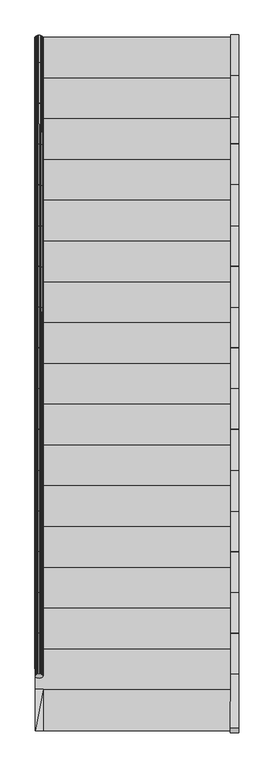
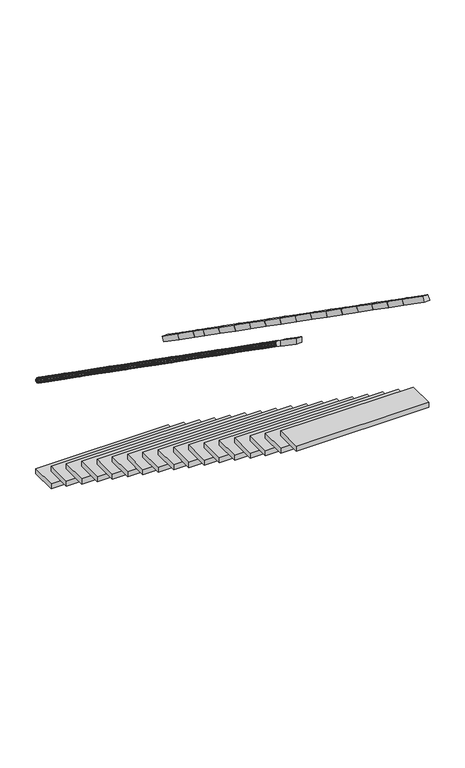
"""IFC4 building model written with IfcOpenShell, lengths in millimetres: stair geometry, 0_3d."""

from ifc_helpers import new_model, si_unit, frame, origin, origin_with_axes, place, context, project, spatial, polyline, outline, extrude, faceted_brep, source, transform, mapped, element, save


def stair_8f8480cc(model_context):
    return source(origin(), model_context, "Body", "SolidModel", [
        extrude(outline(polyline([(8.0820225, -49.3424859), (0.0, 0.0), (301.246492, 49.3424859), (309.3285145, 0.0), (8.0820225, -49.3424859)])), frame((1249.6426286, 1832.7635324, 2592.2240094), z_axis=(8.41828831730923e-05, 0.5732803643846047, 0.8193592720683017), x_axis=(-0.16175918326000965, -0.8085607216158117, 0.5657415718251334)), (0.0, 0.0, 1.0), 50.0),
        extrude(outline(polyline([(1249.9265282, 3766.1029394), (1249.8897991, 3515.9797843), (0.1101896, 3516.5348933), (0.0734597, 3766.4117944), (1249.9265282, 3766.1029394)])), frame((0.0, 0.0, 350.0), z_axis=(0.0, 0.0, 1.0), x_axis=(1.0, 0.0, 0.0)), (0.0, 0.0, 1.0), 50.0),
        faceted_brep([(1.5427287, 2095.0138491, 2432.7450302), (0.3185352, 2099.1390121, 2438.6355957), (1.5415159, 2103.2645348, 2444.5261612), (5.0919569, 2106.9865824, 2449.8401171), (10.6223163, 2109.9408148, 2454.0572963), (17.5912439, 2111.8380512, 2456.7648921), (25.3165726, 2112.4925769, 2457.697866), (33.0420935, 2111.8403223, 2456.7648921), (40.0115786, 2109.9451348, 2454.0572963), (45.5428062, 2106.9925283, 2449.8401171), (49.0943412, 2103.2715247, 2444.5261612), (50.3185347, 2099.1463617, 2438.6355957), (49.095554, 2095.0208389, 2432.7450302), (45.545113, 2091.2987914, 2427.4310744), (40.0147537, 2088.344559, 2423.2138951), (33.045826, 2086.4473226, 2420.5062993), (25.3204973, 2085.7927969, 2419.5733254), (17.5949765, 2086.4450514, 2420.5062993), (10.6254914, 2088.340239, 2423.2138951), (5.0942637, 2091.2928454, 2427.4310744), (0.3552659, 1849.2569855, 2613.6356001), (1.5782465, 1853.3825079, 2619.5261658), (5.1286875, 1857.1045552, 2624.8401219), (10.6590469, 1860.0587874, 2629.0573013), (17.6279745, 1861.9560236, 2631.7648972), (25.3533033, 1862.6105493, 2632.6978712), (33.0788241, 1861.9582948, 2631.7648972), (40.0483092, 1860.0631074, 2629.0573013), (45.5795368, 1857.1105012, 2624.8401219), (49.1310718, 1853.3894978, 2619.5261658), (50.3552653, 1849.2643351, 2613.6356001), (49.1322846, 1845.1388127, 2607.7450345), (45.5818436, 1841.4167654, 2602.4310784), (40.0514843, 1838.4625333, 2598.213899), (33.0825566, 1836.565297, 2595.5063031), (25.3572279, 1835.9107713, 2594.5733291), (17.6317071, 1836.5630258, 2595.5063031), (10.662222, 1838.4582133, 2598.213899), (5.1309944, 1841.4108195, 2602.4310784), (1.5794593, 1845.1318228, 2607.7450345)], [[[0, 1, 2, 3, 4, 5, 6, 7, 8, 9, 10, 11, 12, 13, 14, 15, 16, 17, 18, 19]], [[2, 1, 20, 21]], [[3, 2, 21, 22]], [[4, 3, 22, 23]], [[5, 4, 23, 24]], [[6, 5, 24, 25]], [[7, 6, 25, 26]], [[8, 7, 26, 27]], [[9, 8, 27, 28]], [[10, 9, 28, 29]], [[11, 10, 29, 30]], [[12, 11, 30, 31]], [[13, 12, 31, 32]], [[14, 13, 32, 33]], [[15, 14, 33, 34]], [[16, 15, 34, 35]], [[17, 16, 35, 36]], [[18, 17, 36, 37]], [[19, 18, 37, 38]], [[0, 19, 38, 39]], [[1, 0, 39, 20]], [[21, 20, 39, 38, 37, 36, 35, 34, 33, 32, 31, 30, 29, 28, 27, 26, 25, 24, 23, 22]]]),
        extrude(outline(polyline([(1249.5959661, 1514.9945425), (1249.5592369, 1264.8713869), (0.4407586, 1267.6414831), (0.4040287, 1517.5186441), (1249.5959661, 1514.9945425)])), frame((0.0, 0.0, 1925.0), z_axis=(0.0, 0.0, 1.0), x_axis=(1.0, 0.0, 0.0)), (0.0, 0.0, 1.0), 50.0),
        extrude(outline(polyline([(1249.7061535, 2265.3640086), (1249.6694243, 2015.2408533), (0.3305689, 2017.2728797), (0.293839, 2267.1499541), (1249.7061535, 2265.3640086)])), frame((0.0, 0.0, 1400.0), z_axis=(0.0, 0.0, 1.0), x_axis=(1.0, 0.0, 0.0)), (0.0, 0.0, 1.0), 50.0),
        extrude(outline(polyline([(1249.6694243, 2015.2408533), (1249.6326952, 1765.1176979), (0.3672988, 1767.3957763), (0.3305689, 2017.2728797), (1249.6694243, 2015.2408533)])), frame((0.0, 0.0, 1575.0), z_axis=(0.0, 0.0, 1.0), x_axis=(1.0, 0.0, 0.0)), (0.0, 0.0, 1.0), 50.0),
        faceted_brep([(1.5794593, 1845.1318228, 2607.7450345), (0.3552659, 1849.2569855, 2613.6356001), (1.5782465, 1853.3825079, 2619.5261658), (5.1286875, 1857.1045552, 2624.8401219), (10.6590469, 1860.0587874, 2629.0573013), (17.6279745, 1861.9560236, 2631.7648972), (25.3533033, 1862.6105493, 2632.6978712), (33.0788241, 1861.9582948, 2631.7648972), (40.0483092, 1860.0631074, 2629.0573013), (45.5795368, 1857.1105012, 2624.8401219), (49.1310718, 1853.3894978, 2619.5261658), (50.3552653, 1849.2643351, 2613.6356001), (49.1322846, 1845.1388127, 2607.7450345), (45.5818436, 1841.4167654, 2602.4310784), (40.0514843, 1838.4625333, 2598.213899), (33.0825566, 1836.565297, 2595.5063031), (25.3572279, 1835.9107713, 2594.5733291), (17.6317071, 1836.5630258, 2595.5063031), (10.662222, 1838.4582133, 2598.213899), (5.1309944, 1841.4108195, 2602.4310784), (0.3919965, 1599.3749301, 2788.6356046), (1.6149772, 1603.5004522, 2794.5261705), (5.1654181, 1607.2224992, 2799.8401268), (10.6957775, 1610.1767311, 2804.0573064), (17.6647052, 1612.0739672, 2806.7649023), (25.3900339, 1612.7284928, 2807.6978763), (33.1155547, 1612.0762384, 2806.7649023), (40.0850398, 1610.1810511, 2804.0573064), (45.6162674, 1607.2284451, 2799.8401268), (49.1678025, 1603.5074421, 2794.5261705), (50.3919959, 1599.3822797, 2788.6356046), (49.1690153, 1595.2567576, 2782.7450387), (45.6185743, 1591.5347106, 2777.4310824), (40.0882149, 1588.5804787, 2773.2139028), (33.1192873, 1586.6832425, 2770.5063068), (25.3939585, 1586.0287169, 2769.5733329), (17.6684377, 1586.6809714, 2770.5063068), (10.6989526, 1588.5761587, 2773.2139028), (5.167725, 1591.5287647, 2777.4310824), (1.6161899, 1595.2497677, 2782.7450387)], [[[0, 1, 2, 3, 4, 5, 6, 7, 8, 9, 10, 11, 12, 13, 14, 15, 16, 17, 18, 19]], [[2, 1, 20, 21]], [[3, 2, 21, 22]], [[4, 3, 22, 23]], [[5, 4, 23, 24]], [[6, 5, 24, 25]], [[7, 6, 25, 26]], [[8, 7, 26, 27]], [[9, 8, 27, 28]], [[10, 9, 28, 29]], [[11, 10, 29, 30]], [[12, 11, 30, 31]], [[13, 12, 31, 32]], [[14, 13, 32, 33]], [[15, 14, 33, 34]], [[16, 15, 34, 35]], [[17, 16, 35, 36]], [[18, 17, 36, 37]], [[19, 18, 37, 38]], [[0, 19, 38, 39]], [[1, 0, 39, 20]], [[21, 20, 39, 38, 37, 36, 35, 34, 33, 32, 31, 30, 29, 28, 27, 26, 25, 24, 23, 22]]]),
        faceted_brep([(1.3223451, 3594.3053999, 1382.7450049), (0.0981516, 3598.4305649, 1388.635569), (1.3211323, 3602.5560896, 1394.5261331), (4.8715733, 3606.2781388, 1399.8400878), (10.4019326, 3609.2323726, 1404.0572661), (17.3708603, 3611.1296099, 1406.7648612), (25.096189, 3611.7841359, 1407.6978349), (32.8217098, 3611.1318811, 1406.7648612), (39.7911949, 3609.2366926, 1404.0572661), (45.3224225, 3606.2840848, 1399.8400878), (48.8739576, 3602.5630794, 1394.5261331), (50.0981511, 3598.4379145, 1388.635569), (48.8751704, 3594.3123898, 1382.7450049), (45.3247294, 3590.5903405, 1377.4310502), (39.79437, 3587.6361067, 1373.2138719), (32.8254424, 3585.7388695, 1370.5062768), (25.1001137, 3585.0843435, 1369.5733031), (17.3745928, 3585.7365983, 1370.5062768), (10.4051077, 3587.6317868, 1373.2138719), (4.8738801, 3590.5843946, 1377.4310502), (0.1348822, 3348.5487117, 1563.6355734), (1.3578629, 3352.674236, 1569.5261378), (4.9083039, 3356.396285, 1574.8400927), (10.4386632, 3359.3505186, 1579.0572711), (17.4075909, 3361.2477557, 1581.7648664), (25.1329196, 3361.9022817, 1582.6978401), (32.8584404, 3361.2500269, 1581.7648664), (39.8279255, 3359.3548385, 1579.0572711), (45.3591531, 3356.402231, 1574.8400927), (48.9106882, 3352.6812259, 1569.5261378), (50.1348816, 3348.5560613, 1563.6355734), (48.911901, 3344.4305369, 1557.7450091), (45.36146, 3340.7084879, 1552.4310542), (39.8311006, 3337.7542544, 1548.2138758), (32.862173, 3335.8570172, 1545.5062805), (25.1368442, 3335.2024913, 1544.5733068), (17.4113234, 3335.8547461, 1545.5062805), (10.4418383, 3337.7499344, 1548.2138758), (4.9106107, 3340.702542, 1552.4310542), (1.3590757, 3344.423547, 1557.7450091)], [[[0, 1, 2, 3, 4, 5, 6, 7, 8, 9, 10, 11, 12, 13, 14, 15, 16, 17, 18, 19]], [[2, 1, 20, 21]], [[3, 2, 21, 22]], [[4, 3, 22, 23]], [[5, 4, 23, 24]], [[6, 5, 24, 25]], [[7, 6, 25, 26]], [[8, 7, 26, 27]], [[9, 8, 27, 28]], [[10, 9, 28, 29]], [[11, 10, 29, 30]], [[12, 11, 30, 31]], [[13, 12, 31, 32]], [[14, 13, 32, 33]], [[15, 14, 33, 34]], [[16, 15, 34, 35]], [[17, 16, 35, 36]], [[18, 17, 36, 37]], [[19, 18, 37, 38]], [[0, 19, 38, 39]], [[1, 0, 39, 20]], [[21, 20, 39, 38, 37, 36, 35, 34, 33, 32, 31, 30, 29, 28, 27, 26, 25, 24, 23, 22]]]),
        faceted_brep([(1.4692675, 2594.7778149, 2082.7450218), (0.245074, 2598.9029786, 2088.6355868), (1.4680547, 2603.028502, 2094.5261518), (5.0184957, 2606.7505501, 2099.8401073), (10.548855, 2609.704783, 2104.0572862), (17.5177827, 2611.6020197, 2106.7648818), (25.2431114, 2612.2565455, 2107.6978556), (32.9686322, 2611.6042908, 2106.7648818), (39.9381173, 2609.709103, 2104.0572862), (45.4693449, 2606.7564961, 2099.8401073), (49.02088, 2603.0354919, 2094.5261518), (50.2450735, 2598.9103282, 2088.6355868), (49.0220928, 2594.7848048, 2082.7450218), (45.4716518, 2591.0627567, 2077.4310663), (39.9412924, 2588.1085238, 2073.2138874), (32.9723648, 2586.2112871, 2070.5062918), (25.2470361, 2585.5567613, 2069.573318), (17.5215152, 2586.209016, 2070.5062918), (10.5520301, 2588.1042038, 2073.2138874), (5.0208025, 2591.0568107, 2077.4310663), (0.2818046, 2349.0210098, 2263.6355913), (1.5047853, 2353.1465328, 2269.5261565), (5.0552263, 2356.8685807, 2274.8401122), (10.5855856, 2359.8228133, 2279.0572913), (17.5545133, 2361.7200499, 2281.7648869), (25.279842, 2362.3745756, 2282.6978608), (33.0053628, 2361.722321, 2281.7648869), (39.9748479, 2359.8271333, 2279.0572913), (45.5060756, 2356.8745266, 2274.8401122), (49.0576106, 2353.1535227, 2269.5261565), (50.2818041, 2349.0283594, 2263.6355913), (49.0588234, 2344.9028363, 2257.745026), (45.5083824, 2341.1807885, 2252.4310703), (39.978023, 2338.2265558, 2248.2138912), (33.0090954, 2336.3293193, 2245.5062956), (25.2837667, 2335.6747935, 2244.5733217), (17.5582459, 2336.3270481, 2245.5062956), (10.5887608, 2338.2222359, 2248.2138912), (5.0575331, 2341.1748425, 2252.4310703), (1.5059981, 2344.8958464, 2257.745026)], [[[0, 1, 2, 3, 4, 5, 6, 7, 8, 9, 10, 11, 12, 13, 14, 15, 16, 17, 18, 19]], [[2, 1, 20, 21]], [[3, 2, 21, 22]], [[4, 3, 22, 23]], [[5, 4, 23, 24]], [[6, 5, 24, 25]], [[7, 6, 25, 26]], [[8, 7, 26, 27]], [[9, 8, 27, 28]], [[10, 9, 28, 29]], [[11, 10, 29, 30]], [[12, 11, 30, 31]], [[13, 12, 31, 32]], [[14, 13, 32, 33]], [[15, 14, 33, 34]], [[16, 15, 34, 35]], [[17, 16, 35, 36]], [[18, 17, 36, 37]], [[19, 18, 37, 38]], [[0, 19, 38, 39]], [[1, 0, 39, 20]], [[21, 20, 39, 38, 37, 36, 35, 34, 33, 32, 31, 30, 29, 28, 27, 26, 25, 24, 23, 22]]]),
        extrude(outline(polyline([(1249.7796117, 2765.610319), (1249.7428826, 2515.4871638), (0.2571091, 2517.0269998), (0.2203792, 2766.9040165), (1249.7796117, 2765.610319)])), frame((0.0, 0.0, 1050.0), z_axis=(0.0, 0.0, 1.0), x_axis=(1.0, 0.0, 0.0)), (0.0, 0.0, 1.0), 50.0),
        extrude(outline(polyline([(1249.8897991, 3515.9797843), (1249.85307, 3265.8566293), (0.1469195, 3266.6579632), (0.1101896, 3516.5348933), (1249.8897991, 3515.9797843)])), frame((0.0, 0.0, 525.0), z_axis=(0.0, 0.0, 1.0), x_axis=(1.0, 0.0, 0.0)), (0.0, 0.0, 1.0), 50.0),
        extrude(outline(polyline([(8.0820225, -49.3424858), (0.0, 0.0), (301.2464918, 49.3424859), (309.3285142, 1e-07), (8.0820225, -49.3424858)])), frame((1249.862999, 3333.4729058, 1542.2240093), z_axis=(8.418288315989453e-05, 0.5732803648726768, 0.8193592717268128), x_axis=(-0.1617591834003618, -0.8085607212599576, 0.5657415722935918)), (0.0, 0.0, 1.0), 50.0),
        extrude(outline(polyline([(8.0820225, -49.3424859), (0.0, 0.0), (301.2464924, 49.3424859), (309.3285148, 0.0), (8.0820225, -49.3424859)])), frame((1249.495715, 832.2906153, 3292.2240094), z_axis=(8.418288310454991e-05, 0.5732803637766174, 0.8193592724936917), x_axis=(-0.16175918308892365, -0.8085607220586004, 0.565741571241215)), (0.0, 0.0, 1.0), 50.0),
        faceted_brep([(0.6244082, 14.2556075, 3867.0), (0.5876783, 268.1325506, 3692.0), (50.5877009, 267.9822577, 3692.0), (50.6244323, 14.2555335, 3867.0), (50.5877009, 267.9822577, 3750.0), (0.5876783, 268.1325506, 3750.0), (0.6244082, 14.2556075, 3925.0), (50.6244323, 14.2555335, 3925.0)], [[[0, 1, 2]], [[3, 0, 2]], [[4, 5, 6]], [[7, 4, 6]], [[4, 2, 1, 5]], [[5, 1, 0, 6]], [[6, 0, 3, 7]], [[7, 3, 2, 4]]]),
        faceted_brep([(1.6896512, 1095.4855709, 3132.7450471), (0.4654577, 1099.6107327, 3138.6356135), (1.6884384, 1103.7362542, 3144.5261798), (5.2388794, 1107.4583006, 3149.8401365), (10.7692388, 1110.4125321, 3154.0573164), (17.7381664, 1112.3097679, 3156.7649126), (25.4634951, 1112.9642934, 3157.6978867), (33.189016, 1112.312039, 3156.7649126), (40.1585011, 1110.416852, 3154.0573164), (45.6897287, 1107.4642465, 3149.8401365), (49.2412637, 1103.743244, 3144.5261798), (50.4654572, 1099.6180823, 3138.6356135), (49.2424765, 1095.4925608, 3132.7450471), (45.6920355, 1091.7705144, 3127.4310904), (40.1616762, 1088.8162829, 3123.2139105), (33.1927485, 1086.9190471, 3120.5063144), (25.4674198, 1086.2645216, 3119.5733403), (17.741899, 1086.916776, 3120.5063144), (10.7724139, 1088.811963, 3123.2139105), (5.2411863, 1091.7645685, 3127.4310904), (0.5021884, 849.7285907, 3313.6356179), (1.7251691, 853.8541119, 3319.5261845), (5.27561, 857.576158, 3324.8401414), (10.8059694, 860.5303893, 3329.0573215), (17.7748971, 862.4276249, 3331.7649177), (25.5002258, 863.0821504, 3332.6978918), (33.2257466, 862.4298961, 3331.7649177), (40.1952317, 860.5347092, 3329.0573215), (45.7264593, 857.5821039, 3324.8401414), (49.2779944, 853.8611018, 3319.5261845), (50.5021878, 849.7359403, 3313.6356179), (49.2792072, 845.6104192, 3307.7450513), (45.7287662, 841.8883731, 3302.4310944), (40.1984068, 838.9341418, 3298.2139144), (33.2294792, 837.0369061, 3295.5063181), (25.5041504, 836.3823807, 3294.573344), (17.7786296, 837.034635, 3295.5063181), (10.8091445, 838.9298218, 3298.2139144), (5.2779169, 841.8824271, 3302.4310944), (1.7263819, 845.6034293, 3307.7450513)], [[[0, 1, 2, 3, 4, 5, 6, 7, 8, 9, 10, 11, 12, 13, 14, 15, 16, 17, 18, 19]], [[2, 1, 20, 21]], [[3, 2, 21, 22]], [[4, 3, 22, 23]], [[5, 4, 23, 24]], [[6, 5, 24, 25]], [[7, 6, 25, 26]], [[8, 7, 26, 27]], [[9, 8, 27, 28]], [[10, 9, 28, 29]], [[11, 10, 29, 30]], [[12, 11, 30, 31]], [[13, 12, 31, 32]], [[14, 13, 32, 33]], [[15, 14, 33, 34]], [[16, 15, 34, 35]], [[17, 16, 35, 36]], [[18, 17, 36, 37]], [[19, 18, 37, 38]], [[0, 19, 38, 39]], [[1, 0, 39, 20]], [[21, 20, 39, 38, 37, 36, 35, 34, 33, 32, 31, 30, 29, 28, 27, 26, 25, 24, 23, 22]]]),
        faceted_brep([(1.6161899, 1595.2497677, 2782.7450387), (0.3919965, 1599.3749301, 2788.6356046), (1.6149772, 1603.5004522, 2794.5261705), (5.1654181, 1607.2224992, 2799.8401268), (10.6957775, 1610.1767311, 2804.0573064), (17.6647052, 1612.0739672, 2806.7649023), (25.3900339, 1612.7284928, 2807.6978763), (33.1155547, 1612.0762384, 2806.7649023), (40.0850398, 1610.1810511, 2804.0573064), (45.6162674, 1607.2284451, 2799.8401268), (49.1678025, 1603.5074421, 2794.5261705), (50.3919959, 1599.3822797, 2788.6356046), (49.1690153, 1595.2567576, 2782.7450387), (45.6185743, 1591.5347106, 2777.4310824), (40.0882149, 1588.5804787, 2773.2139028), (33.1192873, 1586.6832425, 2770.5063068), (25.3939585, 1586.0287169, 2769.5733329), (17.6684377, 1586.6809714, 2770.5063068), (10.6989526, 1588.5761587, 2773.2139028), (5.167725, 1591.5287647, 2777.4310824), (0.4287271, 1349.4928458, 2963.635609), (1.6517078, 1353.6183676, 2969.5261752), (5.2021488, 1357.3404143, 2974.8401317), (10.7325081, 1360.294646, 2979.0573114), (17.7014358, 1362.191882, 2981.7649075), (25.4267645, 1362.8464075, 2982.6978815), (33.1522853, 1362.1941531, 2981.7649075), (40.1217704, 1360.298966, 2979.0573114), (45.6529981, 1357.3463602, 2974.8401317), (49.2045331, 1353.6253575, 2969.5261752), (50.4287266, 1349.5001954, 2963.635609), (49.2057459, 1345.3746736, 2957.7450429), (45.6553049, 1341.6526269, 2952.4310864), (40.1249455, 1338.6983952, 2948.2139067), (33.1560179, 1336.8011593, 2945.5063106), (25.4306892, 1336.1466337, 2944.5733366), (17.7051683, 1336.7988881, 2945.5063106), (10.7356832, 1338.6940752, 2948.2139067), (5.2044556, 1341.646681, 2952.4310864), (1.6529206, 1345.3676837, 2957.7450429)], [[[0, 1, 2, 3, 4, 5, 6, 7, 8, 9, 10, 11, 12, 13, 14, 15, 16, 17, 18, 19]], [[2, 1, 20, 21]], [[3, 2, 21, 22]], [[4, 3, 22, 23]], [[5, 4, 23, 24]], [[6, 5, 24, 25]], [[7, 6, 25, 26]], [[8, 7, 26, 27]], [[9, 8, 27, 28]], [[10, 9, 28, 29]], [[11, 10, 29, 30]], [[12, 11, 30, 31]], [[13, 12, 31, 32]], [[14, 13, 32, 33]], [[15, 14, 33, 34]], [[16, 15, 34, 35]], [[17, 16, 35, 36]], [[18, 17, 36, 37]], [[19, 18, 37, 38]], [[0, 19, 38, 39]], [[1, 0, 39, 20]], [[21, 20, 39, 38, 37, 36, 35, 34, 33, 32, 31, 30, 29, 28, 27, 26, 25, 24, 23, 22]]]),
        faceted_brep([(1.2856145, 3844.1872239, 1207.7450006), (0.061421, 3848.3123892, 1213.6355645), (1.2844017, 3852.4379142, 1219.5261284), (4.8348427, 3856.1599637, 1224.8400829), (10.365202, 3859.1141977, 1229.057261), (17.3341297, 3861.0114352, 1231.7648561), (25.0594584, 3861.6659612, 1232.6978297), (32.7849792, 3861.0137063, 1231.7648561), (39.7544643, 3859.1185177, 1229.057261), (45.2856919, 3856.1659097, 1224.8400829), (48.837227, 3852.444904, 1219.5261284), (50.0614205, 3848.3197388, 1213.6355645), (48.8384398, 3844.1942138, 1207.7450006), (45.2879988, 3840.4721642, 1202.4310462), (39.7576394, 3837.5179302, 1198.213868), (32.7887118, 3835.6206928, 1195.506273), (25.0633831, 3834.9661667, 1194.5732993), (17.3378622, 3835.6184216, 1195.506273), (10.3683771, 3837.5136102, 1198.213868), (4.8371495, 3840.4662183, 1202.4310462), (0.0981516, 3598.4305649, 1388.635569), (1.3211323, 3602.5560896, 1394.5261331), (4.8715733, 3606.2781388, 1399.8400878), (10.4019326, 3609.2323726, 1404.0572661), (17.3708603, 3611.1296099, 1406.7648612), (25.096189, 3611.7841359, 1407.6978349), (32.8217098, 3611.1318811, 1406.7648612), (39.7911949, 3609.2366926, 1404.0572661), (45.3224225, 3606.2840848, 1399.8400878), (48.8739576, 3602.5630794, 1394.5261331), (50.0981511, 3598.4379145, 1388.635569), (48.8751704, 3594.3123898, 1382.7450049), (45.3247294, 3590.5903405, 1377.4310502), (39.79437, 3587.6361067, 1373.2138719), (32.8254424, 3585.7388695, 1370.5062768), (25.1001137, 3585.0843435, 1369.5733031), (17.3745928, 3585.7365983, 1370.5062768), (10.4051077, 3587.6317868, 1373.2138719), (4.8738801, 3590.5843946, 1377.4310502), (1.3223451, 3594.3053999, 1382.7450049)], [[[0, 1, 2, 3, 4, 5, 6, 7, 8, 9, 10, 11, 12, 13, 14, 15, 16, 17, 18, 19]], [[2, 1, 20, 21]], [[3, 2, 21, 22]], [[4, 3, 22, 23]], [[5, 4, 23, 24]], [[6, 5, 24, 25]], [[7, 6, 25, 26]], [[8, 7, 26, 27]], [[9, 8, 27, 28]], [[10, 9, 28, 29]], [[11, 10, 29, 30]], [[12, 11, 30, 31]], [[13, 12, 31, 32]], [[14, 13, 32, 33]], [[15, 14, 33, 34]], [[16, 15, 34, 35]], [[17, 16, 35, 36]], [[18, 17, 36, 37]], [[19, 18, 37, 38]], [[0, 19, 38, 39]], [[1, 0, 39, 20]], [[21, 20, 39, 38, 37, 36, 35, 34, 33, 32, 31, 30, 29, 28, 27, 26, 25, 24, 23, 22]]]),
        faceted_brep([(1.4325369, 2844.6597545, 1907.7450176), (0.2083434, 2848.7849185, 1913.6355824), (1.4313241, 2852.9104422, 1919.5261472), (4.9817651, 2856.6324906, 1924.8401024), (10.5121244, 2859.5867237, 1929.0572812), (17.4810521, 2861.4839606, 1931.7648767), (25.2063808, 2862.1384864, 1932.6978505), (32.9319016, 2861.4862317, 1931.7648767), (39.9013867, 2859.5910437, 1929.0572812), (45.4326143, 2856.6384366, 1924.8401024), (48.9841494, 2852.9174321, 1919.5261472), (50.2083429, 2848.7922681, 1913.6355824), (48.9853622, 2844.6667444, 1907.7450176), (45.4349212, 2840.944696, 1902.4310623), (39.9045618, 2837.9904629, 1898.2138835), (32.9356342, 2836.093226, 1895.5062881), (25.2103054, 2835.4387002, 1894.5733142), (17.4847846, 2836.0909549, 1895.5062881), (10.5152995, 2837.9861429, 1898.2138835), (4.9840719, 2840.9387501, 1902.4310623), (0.245074, 2598.9029786, 2088.6355868), (1.4680547, 2603.028502, 2094.5261518), (5.0184957, 2606.7505501, 2099.8401073), (10.548855, 2609.704783, 2104.0572862), (17.5177827, 2611.6020197, 2106.7648818), (25.2431114, 2612.2565455, 2107.6978556), (32.9686322, 2611.6042908, 2106.7648818), (39.9381173, 2609.709103, 2104.0572862), (45.4693449, 2606.7564961, 2099.8401073), (49.02088, 2603.0354919, 2094.5261518), (50.2450735, 2598.9103282, 2088.6355868), (49.0220928, 2594.7848048, 2082.7450218), (45.4716518, 2591.0627567, 2077.4310663), (39.9412924, 2588.1085238, 2073.2138874), (32.9723648, 2586.2112871, 2070.5062918), (25.2470361, 2585.5567613, 2069.573318), (17.5215152, 2586.209016, 2070.5062918), (10.5520301, 2588.1042038, 2073.2138874), (5.0208025, 2591.0568107, 2077.4310663), (1.4692675, 2594.7778149, 2082.7450218)], [[[0, 1, 2, 3, 4, 5, 6, 7, 8, 9, 10, 11, 12, 13, 14, 15, 16, 17, 18, 19]], [[2, 1, 20, 21]], [[3, 2, 21, 22]], [[4, 3, 22, 23]], [[5, 4, 23, 24]], [[6, 5, 24, 25]], [[7, 6, 25, 26]], [[8, 7, 26, 27]], [[9, 8, 27, 28]], [[10, 9, 28, 29]], [[11, 10, 29, 30]], [[12, 11, 30, 31]], [[13, 12, 31, 32]], [[14, 13, 32, 33]], [[15, 14, 33, 34]], [[16, 15, 34, 35]], [[17, 16, 35, 36]], [[18, 17, 36, 37]], [[19, 18, 37, 38]], [[0, 19, 38, 39]], [[1, 0, 39, 20]], [[21, 20, 39, 38, 37, 36, 35, 34, 33, 32, 31, 30, 29, 28, 27, 26, 25, 24, 23, 22]]]),
        extrude(outline(polyline([(8.0820224, -49.3424858), (0.0, 0.0), (301.2464917, 49.3424859), (309.3285142, 1e-07), (8.0820224, -49.3424858)])), frame((1249.8997274, 3583.5911345, 1367.2240093), z_axis=(8.418288314084033e-05, 0.5732803649046162, 0.8193592717044657), x_axis=(-0.1617591834100128, -0.8085607212366094, 0.5657415723242016)), (0.0, 0.0, 1.0), 50.0),
        extrude(outline(polyline([(1249.5592369, 1264.8713869), (1249.5225078, 1014.7482313), (0.4774885, 1017.7642932), (0.4407586, 1267.6414831), (1249.5592369, 1264.8713869)])), frame((0.0, 0.0, 2100.0), z_axis=(0.0, 0.0, 1.0), x_axis=(1.0, 0.0, 0.0)), (0.0, 0.0, 1.0), 50.0),
        faceted_brep([(1.3590757, 3344.423547, 1557.7450091), (0.1348822, 3348.5487117, 1563.6355734), (1.3578629, 3352.674236, 1569.5261378), (4.9083039, 3356.396285, 1574.8400927), (10.4386632, 3359.3505186, 1579.0572711), (17.4075909, 3361.2477557, 1581.7648664), (25.1329196, 3361.9022817, 1582.6978401), (32.8584404, 3361.2500269, 1581.7648664), (39.8279255, 3359.3548385, 1579.0572711), (45.3591531, 3356.402231, 1574.8400927), (48.9106882, 3352.6812259, 1569.5261378), (50.1348816, 3348.5560613, 1563.6355734), (48.911901, 3344.4305369, 1557.7450091), (45.36146, 3340.7084879, 1552.4310542), (39.8311006, 3337.7542544, 1548.2138758), (32.862173, 3335.8570172, 1545.5062805), (25.1368442, 3335.2024913, 1544.5733068), (17.4113234, 3335.8547461, 1545.5062805), (10.4418383, 3337.7499344, 1548.2138758), (4.9106107, 3340.702542, 1552.4310542), (0.1716128, 3098.6668296, 1738.6355779), (1.3945935, 3102.7923536, 1744.5261425), (4.9450345, 3106.5144023, 1749.8400975), (10.4753938, 3109.4686356, 1754.0572762), (17.4443215, 3111.3658726, 1756.7648715), (25.1696502, 3112.0203985, 1757.6978453), (32.895171, 3111.3681438, 1756.7648715), (39.8646561, 3109.4729556, 1754.0572762), (45.3958837, 3106.5203482, 1749.8400975), (48.9474188, 3102.7993435, 1744.5261425), (50.1716122, 3098.6741791, 1738.6355779), (48.9486316, 3094.5486551, 1732.7450133), (45.3981906, 3090.8266064, 1727.4310583), (39.8678312, 3087.8723731, 1723.2138796), (32.8989036, 3085.9751361, 1720.5062843), (25.1735748, 3085.3206102, 1719.5733105), (17.448054, 3085.9728649, 1720.5062843), (10.4785689, 3087.8680531, 1723.2138796), (4.9473413, 3090.8206605, 1727.4310583), (1.3958063, 3094.5416652, 1732.7450133)], [[[0, 1, 2, 3, 4, 5, 6, 7, 8, 9, 10, 11, 12, 13, 14, 15, 16, 17, 18, 19]], [[2, 1, 20, 21]], [[3, 2, 21, 22]], [[4, 3, 22, 23]], [[5, 4, 23, 24]], [[6, 5, 24, 25]], [[7, 6, 25, 26]], [[8, 7, 26, 27]], [[9, 8, 27, 28]], [[10, 9, 28, 29]], [[11, 10, 29, 30]], [[12, 11, 30, 31]], [[13, 12, 31, 32]], [[14, 13, 32, 33]], [[15, 14, 33, 34]], [[16, 15, 34, 35]], [[17, 16, 35, 36]], [[18, 17, 36, 37]], [[19, 18, 37, 38]], [[0, 19, 38, 39]], [[1, 0, 39, 20]], [[21, 20, 39, 38, 37, 36, 35, 34, 33, 32, 31, 30, 29, 28, 27, 26, 25, 24, 23, 22]]]),
        extrude(outline(polyline([(1249.4857787, 764.6250755), (1249.4490496, 514.5019196), (0.5509483, 518.0098269), (0.5142184, 767.8870744), (1249.4857787, 764.6250755)])), frame((0.0, 0.0, 2450.0), z_axis=(0.0, 0.0, 1.0), x_axis=(1.0, 0.0, 0.0)), (0.0, 0.0, 1.0), 50.0),
        extrude(outline(polyline([(8.0820225, -49.3424859), (0.0, 0.0), (301.246492, 49.3424859), (309.3285144, 0.0), (8.0820225, -49.3424859)])), frame((1249.679357, 2082.8817614, 2417.2240094), z_axis=(8.418288319098076e-05, 0.5732803645012542, 0.8193592719866855), x_axis=(-0.16175918329309924, -0.8085607215308216, 0.5657415719371407)), (0.0, 0.0, 1.0), 50.0),
        faceted_brep([(1.6529206, 1345.3676837, 2957.7450429), (0.4287271, 1349.4928458, 2963.635609), (1.6517078, 1353.6183676, 2969.5261752), (5.2021488, 1357.3404143, 2974.8401317), (10.7325081, 1360.294646, 2979.0573114), (17.7014358, 1362.191882, 2981.7649075), (25.4267645, 1362.8464075, 2982.6978815), (33.1522853, 1362.1941531, 2981.7649075), (40.1217704, 1360.298966, 2979.0573114), (45.6529981, 1357.3463602, 2974.8401317), (49.2045331, 1353.6253575, 2969.5261752), (50.4287266, 1349.5001954, 2963.635609), (49.2057459, 1345.3746736, 2957.7450429), (45.6553049, 1341.6526269, 2952.4310864), (40.1249455, 1338.6983952, 2948.2139067), (33.1560179, 1336.8011593, 2945.5063106), (25.4306892, 1336.1466337, 2944.5733366), (17.7051683, 1336.7988881, 2945.5063106), (10.7356832, 1338.6940752, 2948.2139067), (5.2044556, 1341.646681, 2952.4310864), (0.4654577, 1099.6107327, 3138.6356135), (1.6884384, 1103.7362542, 3144.5261798), (5.2388794, 1107.4583006, 3149.8401365), (10.7692388, 1110.4125321, 3154.0573164), (17.7381664, 1112.3097679, 3156.7649126), (25.4634951, 1112.9642934, 3157.6978867), (33.189016, 1112.312039, 3156.7649126), (40.1585011, 1110.416852, 3154.0573164), (45.6897287, 1107.4642465, 3149.8401365), (49.2412637, 1103.743244, 3144.5261798), (50.4654572, 1099.6180823, 3138.6356135), (49.2424765, 1095.4925608, 3132.7450471), (45.6920355, 1091.7705144, 3127.4310904), (40.1616762, 1088.8162829, 3123.2139105), (33.1927485, 1086.9190471, 3120.5063144), (25.4674198, 1086.2645216, 3119.5733403), (17.741899, 1086.916776, 3120.5063144), (10.7724139, 1088.811963, 3123.2139105), (5.2411863, 1091.7645685, 3127.4310904), (1.6896512, 1095.4855709, 3132.7450471)], [[[0, 1, 2, 3, 4, 5, 6, 7, 8, 9, 10, 11, 12, 13, 14, 15, 16, 17, 18, 19]], [[2, 1, 20, 21]], [[3, 2, 21, 22]], [[4, 3, 22, 23]], [[5, 4, 23, 24]], [[6, 5, 24, 25]], [[7, 6, 25, 26]], [[8, 7, 26, 27]], [[9, 8, 27, 28]], [[10, 9, 28, 29]], [[11, 10, 29, 30]], [[12, 11, 30, 31]], [[13, 12, 31, 32]], [[14, 13, 32, 33]], [[15, 14, 33, 34]], [[16, 15, 34, 35]], [[17, 16, 35, 36]], [[18, 17, 36, 37]], [[19, 18, 37, 38]], [[0, 19, 38, 39]], [[1, 0, 39, 20]], [[21, 20, 39, 38, 37, 36, 35, 34, 33, 32, 31, 30, 29, 28, 27, 26, 25, 24, 23, 22]]]),
        extrude(outline(polyline([(8.0820225, -49.3424859), (0.0, 0.0), (301.2464922, 49.3424859), (309.3285146, 0.0), (8.0820225, -49.3424859)])), frame((1249.6059002, 1582.6453033, 2767.2240094), z_axis=(8.418288318234878e-05, 0.5732803642537855, 0.8193592721598316), x_axis=(-0.1617591832231551, -0.808560721711089, 0.5657415716995001)), (0.0, 0.0, 1.0), 50.0),
        extrude(outline(polyline([(8.0820225, -49.3424858), (0.0, 0.0), (301.2464918, 49.3424859), (309.3285142, 1e-07), (8.0820225, -49.3424858)])), frame((1249.9611524, 4001.8916658, 1074.5520464), z_axis=(8.41828832501973e-05, 0.5732803649279318, 0.8193592716881524), x_axis=(-0.1617591834181913, -0.8085607212194018, 0.5657415723464564)), (0.0, 0.0, 1.0), 50.0),
        faceted_brep([(1.2488839, 4094.0690189, 1032.7449964), (0.0246904, 4098.1941845, 1038.6355601), (1.2476711, 4102.3197098, 1044.5261238), (4.7981121, 4106.0417597, 1049.840078), (10.3284714, 4108.9959939, 1054.057256), (17.2973991, 4110.8932315, 1056.7648509), (25.0227278, 4111.5477576, 1057.6978246), (32.7482486, 4110.8955027, 1056.7648509), (39.7177337, 4109.0003139, 1054.057256), (45.2489614, 4106.0477056, 1049.840078), (48.8004964, 4102.3266997, 1044.5261238), (50.0246899, 4098.2015341, 1038.6355601), (48.8017092, 4094.0760088, 1032.7449964), (45.2512682, 4090.3539589, 1027.4310421), (39.7209088, 4087.3997247, 1023.2138642), (32.7519812, 4085.5024871, 1020.5062692), (25.0266525, 4084.847961, 1019.5732956), (17.3011317, 4085.500216, 1020.5062692), (10.3316466, 4087.3954047, 1023.2138642), (4.8004189, 4090.348013, 1027.4310421), (0.061421, 3848.3123892, 1213.6355645), (1.2844017, 3852.4379142, 1219.5261284), (4.8348427, 3856.1599637, 1224.8400829), (10.365202, 3859.1141977, 1229.057261), (17.3341297, 3861.0114352, 1231.7648561), (25.0594584, 3861.6659612, 1232.6978297), (32.7849792, 3861.0137063, 1231.7648561), (39.7544643, 3859.1185177, 1229.057261), (45.2856919, 3856.1659097, 1224.8400829), (48.837227, 3852.444904, 1219.5261284), (50.0614205, 3848.3197388, 1213.6355645), (48.8384398, 3844.1942138, 1207.7450006), (45.2879988, 3840.4721642, 1202.4310462), (39.7576394, 3837.5179302, 1198.213868), (32.7887118, 3835.6206928, 1195.506273), (25.0633831, 3834.9661667, 1194.5732993), (17.3378622, 3835.6184216, 1195.506273), (10.3683771, 3837.5136102, 1198.213868), (4.8371495, 3840.4662183, 1202.4310462), (1.2856145, 3844.1872239, 1207.7450006)], [[[0, 1, 2, 3, 4, 5, 6, 7, 8, 9, 10, 11, 12, 13, 14, 15, 16, 17, 18, 19]], [[2, 1, 20, 21]], [[3, 2, 21, 22]], [[4, 3, 22, 23]], [[5, 4, 23, 24]], [[6, 5, 24, 25]], [[7, 6, 25, 26]], [[8, 7, 26, 27]], [[9, 8, 27, 28]], [[10, 9, 28, 29]], [[11, 10, 29, 30]], [[12, 11, 30, 31]], [[13, 12, 31, 32]], [[14, 13, 32, 33]], [[15, 14, 33, 34]], [[16, 15, 34, 35]], [[17, 16, 35, 36]], [[18, 17, 36, 37]], [[19, 18, 37, 38]], [[0, 19, 38, 39]], [[1, 0, 39, 20]], [[21, 20, 39, 38, 37, 36, 35, 34, 33, 32, 31, 30, 29, 28, 27, 26, 25, 24, 23, 22]]]),
        extrude(outline(polyline([(8.0820225, -49.3424858), (0.0, 0.0), (301.2464918, 49.3424859), (309.3285142, 1e-07), (8.0820225, -49.3424858)])), frame((1249.8262706, 3083.354677, 1717.2240093), z_axis=(8.418288321802858e-05, 0.5732803648266481, 0.8193592717590175), x_axis=(-0.16175918338648482, -0.8085607212935979, 0.5657415722494806)), (0.0, 0.0, 1.0), 50.0),
        extrude(outline(polyline([(11.8336015, -48.5794799), (0.0, 0.0), (199.4292167, 48.57948), (211.2628181, 0.0), (11.8336015, -48.5794799)])), frame((1249.924424, 3751.773437, 1249.5520464), z_axis=(8.418288319610166e-05, 0.5732803649196659, 0.8193592716939356), x_axis=(-0.23678892715388222, -0.7960461843199325, 0.5569932462848984)), (0.0, 0.0, 1.0), 50.0),
        extrude(outline(polyline([(8.0820225, -49.3424858), (0.0, 0.0), (301.2464917, 49.3424859), (309.3285142, 1e-07), (8.0820225, -49.3424858)])), frame((1249.9978808, 4252.0098945, 899.5520464), z_axis=(8.418288330599988e-05, 0.5732803649220624, 0.8193592716922591), x_axis=(-0.16175918341661352, -0.8085607212236612, 0.5657415723408199)), (0.0, 0.0, 1.0), 50.0),
        extrude(outline(polyline([(8.0820225, -49.3424858), (0.0, 0.0), (301.2464919, 49.3424859), (309.3285143, 1e-07), (8.0820225, -49.3424858)])), frame((1249.7895422, 2833.2364482, 1892.2240093), z_axis=(8.418288334449686e-05, 0.5732803647665086, 0.8193592718010952), x_axis=(-0.16175918336906983, -0.8085607213374504, 0.5657415721917858)), (0.0, 0.0, 1.0), 50.0),
        extrude(outline(polyline([(1249.6326952, 1765.1176979), (1249.5959661, 1514.9945425), (0.4040287, 1517.5186441), (0.3672988, 1767.3957763), (1249.6326952, 1765.1176979)])), frame((0.0, 0.0, 1750.0), z_axis=(0.0, 0.0, 1.0), x_axis=(1.0, 0.0, 0.0)), (0.0, 0.0, 1.0), 50.0),
        extrude(outline(polyline([(1249.8163409, 3015.7334742), (1249.7796117, 2765.610319), (0.2203792, 2766.9040165), (0.1836493, 3016.7810043), (1249.8163409, 3015.7334742)])), frame((0.0, 0.0, 875.0), z_axis=(0.0, 0.0, 1.0), x_axis=(1.0, 0.0, 0.0)), (0.0, 0.0, 1.0), 50.0),
        extrude(outline(polyline([(6.1224459, -49.6237409), (0.0, 0.0), (402.2110965, 49.6237409), (408.3335424, 0.0), (6.1224459, -49.6237409)])), frame((1249.4222582, 332.0541562, 3642.2240094), z_axis=(8.418288299665011e-05, 0.5732803633712008, 0.819359272777349), x_axis=(-0.12256832832714479, -0.8131754547795876, 0.5689663299661063)), (0.0, 0.0, 1.0), 50.0),
        faceted_brep([(1.7263819, 845.6034293, 3307.7450513), (0.5021884, 849.7285907, 3313.6356179), (1.7251691, 853.8541119, 3319.5261845), (5.27561, 857.576158, 3324.8401414), (10.8059694, 860.5303893, 3329.0573215), (17.7748971, 862.4276249, 3331.7649177), (25.5002258, 863.0821504, 3332.6978918), (33.2257466, 862.4298961, 3331.7649177), (40.1952317, 860.5347092, 3329.0573215), (45.7264593, 857.5821039, 3324.8401414), (49.2779944, 853.8611018, 3319.5261845), (50.5021878, 849.7359403, 3313.6356179), (49.2792072, 845.6104192, 3307.7450513), (45.7287662, 841.8883731, 3302.4310944), (40.1984068, 838.9341418, 3298.2139144), (33.2294792, 837.0369061, 3295.5063181), (25.5041504, 836.3823807, 3294.573344), (17.7786296, 837.034635, 3295.5063181), (10.8091445, 838.9298218, 3298.2139144), (5.2779169, 841.8824271, 3302.4310944), (0.538919, 599.84642, 3488.6356224), (1.7618997, 603.9719408, 3494.5261892), (5.3123407, 607.6939866, 3499.8401463), (10.8427001, 610.6482177, 3504.0573265), (17.8116277, 612.5454532, 3506.7649229), (25.5369564, 613.1999786, 3507.697897), (33.2624772, 612.5477243, 3506.7649229), (40.2319623, 610.6525376, 3504.0573265), (45.76319, 607.6999326, 3499.8401463), (49.314725, 603.9789307, 3494.5261892), (50.5389185, 599.8537696, 3488.6356224), (49.3159378, 595.7282487, 3482.7450556), (45.7654968, 592.0062029, 3477.4310985), (40.2351375, 589.0519719, 3473.2139182), (33.2662098, 587.1547364, 3470.5063219), (25.5408811, 586.500211, 3469.5733477), (17.8153603, 587.1524652, 3470.5063219), (10.8458752, 589.0476519, 3473.2139182), (5.3146475, 592.000257, 3477.4310985), (1.7631125, 595.7212589, 3482.7450556)], [[[0, 1, 2, 3, 4, 5, 6, 7, 8, 9, 10, 11, 12, 13, 14, 15, 16, 17, 18, 19]], [[2, 1, 20, 21]], [[3, 2, 21, 22]], [[4, 3, 22, 23]], [[5, 4, 23, 24]], [[6, 5, 24, 25]], [[7, 6, 25, 26]], [[8, 7, 26, 27]], [[9, 8, 27, 28]], [[10, 9, 28, 29]], [[11, 10, 29, 30]], [[12, 11, 30, 31]], [[13, 12, 31, 32]], [[14, 13, 32, 33]], [[15, 14, 33, 34]], [[16, 15, 34, 35]], [[17, 16, 35, 36]], [[18, 17, 36, 37]], [[19, 18, 37, 38]], [[0, 19, 38, 39]], [[1, 0, 39, 20]], [[21, 20, 39, 38, 37, 36, 35, 34, 33, 32, 31, 30, 29, 28, 27, 26, 25, 24, 23, 22]]]),
        faceted_brep([(1.5059981, 2344.8958464, 2257.745026), (0.2818046, 2349.0210098, 2263.6355913), (1.5047853, 2353.1465328, 2269.5261565), (5.0552263, 2356.8685807, 2274.8401122), (10.5855856, 2359.8228133, 2279.0572913), (17.5545133, 2361.7200499, 2281.7648869), (25.279842, 2362.3745756, 2282.6978608), (33.0053628, 2361.722321, 2281.7648869), (39.9748479, 2359.8271333, 2279.0572913), (45.5060756, 2356.8745266, 2274.8401122), (49.0576106, 2353.1535227, 2269.5261565), (50.2818041, 2349.0283594, 2263.6355913), (49.0588234, 2344.9028363, 2257.745026), (45.5083824, 2341.1807885, 2252.4310703), (39.978023, 2338.2265558, 2248.2138912), (33.0090954, 2336.3293193, 2245.5062956), (25.2837667, 2335.6747935, 2244.5733217), (17.5582459, 2336.3270481, 2245.5062956), (10.5887608, 2338.2222359, 2248.2138912), (5.0575331, 2341.1748425, 2252.4310703), (0.3185352, 2099.1390121, 2438.6355957), (1.5415159, 2103.2645348, 2444.5261612), (5.0919569, 2106.9865824, 2449.8401171), (10.6223163, 2109.9408148, 2454.0572963), (17.5912439, 2111.8380512, 2456.7648921), (25.3165726, 2112.4925769, 2457.697866), (33.0420935, 2111.8403223, 2456.7648921), (40.0115786, 2109.9451348, 2454.0572963), (45.5428062, 2106.9925283, 2449.8401171), (49.0943412, 2103.2715247, 2444.5261612), (50.3185347, 2099.1463617, 2438.6355957), (49.095554, 2095.0208389, 2432.7450302), (45.545113, 2091.2987914, 2427.4310744), (40.0147537, 2088.344559, 2423.2138951), (33.045826, 2086.4473226, 2420.5062993), (25.3204973, 2085.7927969, 2419.5733254), (17.5949765, 2086.4450514, 2420.5062993), (10.6254914, 2088.340239, 2423.2138951), (5.0942637, 2091.2928454, 2427.4310744), (1.5427287, 2095.0138491, 2432.7450302)], [[[0, 1, 2, 3, 4, 5, 6, 7, 8, 9, 10, 11, 12, 13, 14, 15, 16, 17, 18, 19]], [[2, 1, 20, 21]], [[3, 2, 21, 22]], [[4, 3, 22, 23]], [[5, 4, 23, 24]], [[6, 5, 24, 25]], [[7, 6, 25, 26]], [[8, 7, 26, 27]], [[9, 8, 27, 28]], [[10, 9, 28, 29]], [[11, 10, 29, 30]], [[12, 11, 30, 31]], [[13, 12, 31, 32]], [[14, 13, 32, 33]], [[15, 14, 33, 34]], [[16, 15, 34, 35]], [[17, 16, 35, 36]], [[18, 17, 36, 37]], [[19, 18, 37, 38]], [[0, 19, 38, 39]], [[1, 0, 39, 20]], [[21, 20, 39, 38, 37, 36, 35, 34, 33, 32, 31, 30, 29, 28, 27, 26, 25, 24, 23, 22]]]),
        extrude(outline(polyline([(1249.4490496, 514.5019196), (1249.4123204, 264.3787636), (0.5876783, 268.1325506), (0.5509483, 518.0098269), (1249.4490496, 514.5019196)])), frame((0.0, 0.0, 2625.0), z_axis=(0.0, 0.0, 1.0), x_axis=(1.0, 0.0, 0.0)), (0.0, 0.0, 1.0), 50.0),
        extrude(outline(polyline([(8.0820225, -49.3424858), (0.0, 0.0), (301.246492, 49.3424859), (309.3285145, 0.0), (8.0820225, -49.3424858)])), frame((1249.7160854, 2332.9999904, 2242.2240093), z_axis=(8.418288328135293e-05, 0.5732803646038177, 0.819359271914925), x_axis=(-0.16175918332223047, -0.8085607214560823, 0.5657415720356289)), (0.0, 0.0, 1.0), 50.0),
        extrude(outline(polyline([(1249.5225078, 1014.7482313), (1249.4857787, 764.6250755), (0.5142184, 767.8870744), (0.4774885, 1017.7642932), (1249.5225078, 1014.7482313)])), frame((0.0, 0.0, 2275.0), z_axis=(0.0, 0.0, 1.0), x_axis=(1.0, 0.0, 0.0)), (0.0, 0.0, 1.0), 50.0),
        extrude(outline(polyline([(1249.85307, 3265.8566293), (1249.8163409, 3015.7334742), (0.1836493, 3016.7810043), (0.1469195, 3266.6579632), (1249.85307, 3265.8566293)])), frame((0.0, 0.0, 700.0), z_axis=(0.0, 0.0, 1.0), x_axis=(1.0, 0.0, 0.0)), (0.0, 0.0, 1.0), 50.0),
        extrude(outline(polyline([(8.0820225, -49.3424859), (0.0, 0.0), (301.2464925, 49.3424859), (309.3285149, 0.0), (8.0820225, -49.3424859)])), frame((1249.4589866, 582.1723858, 3467.2240094), z_axis=(8.418288308120747e-05, 0.5732803635893051, 0.8193592726247483), x_axis=(-0.16175918303658923, -0.8085607221949673, 0.5657415710612826)), (0.0, 0.0, 1.0), 50.0),
        faceted_brep([(1.3958063, 3094.5416652, 1732.7450133), (0.1716128, 3098.6668296, 1738.6355779), (1.3945935, 3102.7923536, 1744.5261425), (4.9450345, 3106.5144023, 1749.8400975), (10.4753938, 3109.4686356, 1754.0572762), (17.4443215, 3111.3658726, 1756.7648715), (25.1696502, 3112.0203985, 1757.6978453), (32.895171, 3111.3681438, 1756.7648715), (39.8646561, 3109.4729556, 1754.0572762), (45.3958837, 3106.5203482, 1749.8400975), (48.9474188, 3102.7993435, 1744.5261425), (50.1716122, 3098.6741791, 1738.6355779), (48.9486316, 3094.5486551, 1732.7450133), (45.3981906, 3090.8266064, 1727.4310583), (39.8678312, 3087.8723731, 1723.2138796), (32.8989036, 3085.9751361, 1720.5062843), (25.1735748, 3085.3206102, 1719.5733105), (17.448054, 3085.9728649, 1720.5062843), (10.4785689, 3087.8680531, 1723.2138796), (4.9473413, 3090.8206605, 1727.4310583), (0.2083434, 2848.7849185, 1913.6355824), (1.4313241, 2852.9104422, 1919.5261472), (4.9817651, 2856.6324906, 1924.8401024), (10.5121244, 2859.5867237, 1929.0572812), (17.4810521, 2861.4839606, 1931.7648767), (25.2063808, 2862.1384864, 1932.6978505), (32.9319016, 2861.4862317, 1931.7648767), (39.9013867, 2859.5910437, 1929.0572812), (45.4326143, 2856.6384366, 1924.8401024), (48.9841494, 2852.9174321, 1919.5261472), (50.2083429, 2848.7922681, 1913.6355824), (48.9853622, 2844.6667444, 1907.7450176), (45.4349212, 2840.944696, 1902.4310623), (39.9045618, 2837.9904629, 1898.2138835), (32.9356342, 2836.093226, 1895.5062881), (25.2103054, 2835.4387002, 1894.5733142), (17.4847846, 2836.0909549, 1895.5062881), (10.5152995, 2837.9861429, 1898.2138835), (4.9840719, 2840.9387501, 1902.4310623), (1.4325369, 2844.6597545, 1907.7450176)], [[[0, 1, 2, 3, 4, 5, 6, 7, 8, 9, 10, 11, 12, 13, 14, 15, 16, 17, 18, 19]], [[2, 1, 20, 21]], [[3, 2, 21, 22]], [[4, 3, 22, 23]], [[5, 4, 23, 24]], [[6, 5, 24, 25]], [[7, 6, 25, 26]], [[8, 7, 26, 27]], [[9, 8, 27, 28]], [[10, 9, 28, 29]], [[11, 10, 29, 30]], [[12, 11, 30, 31]], [[13, 12, 31, 32]], [[14, 13, 32, 33]], [[15, 14, 33, 34]], [[16, 15, 34, 35]], [[17, 16, 35, 36]], [[18, 17, 36, 37]], [[19, 18, 37, 38]], [[0, 19, 38, 39]], [[1, 0, 39, 20]], [[21, 20, 39, 38, 37, 36, 35, 34, 33, 32, 31, 30, 29, 28, 27, 26, 25, 24, 23, 22]]]),
        extrude(outline(polyline([(8.0820225, -49.3424858), (0.0, 0.0), (301.2464919, 49.3424859), (309.3285143, 1e-07), (8.0820225, -49.3424858)])), frame((1249.7528138, 2583.1182193, 2067.2240093), z_axis=(8.418288341734137e-05, 0.5732803646922456, 0.8193592718530548), x_axis=(-0.16175918334768244, -0.8085607213915934, 0.5657415721205195)), (0.0, 0.0, 1.0), 50.0),
        extrude(outline(polyline([(1249.7428826, 2515.4871638), (1249.7061535, 2265.3640086), (0.293839, 2267.1499541), (0.2571091, 2517.0269998), (1249.7428826, 2515.4871638)])), frame((0.0, 0.0, 1225.0), z_axis=(0.0, 0.0, 1.0), x_axis=(1.0, 0.0, 0.0)), (0.0, 0.0, 1.0), 50.0),
        extrude(outline(polyline([(1249.9999865, 4266.3492495), (1249.9632574, 4016.2260945), (0.0367299, 4016.2886665), (0.0, 4266.1655097), (1249.9999865, 4266.3492495)])), origin_with_axes(), (0.0, 0.0, 1.0), 50.0),
        extrude(outline(polyline([(8.0820224, -49.3424859), (0.0, 0.0), (301.2464922, 49.3424859), (309.3285146, 0.0), (8.0820224, -49.3424859)])), frame((1249.5691718, 1332.527074, 2942.2240094), z_axis=(8.418288311948242e-05, 0.5732803641088847, 0.8193592722612145), x_axis=(-0.16175918318212845, -0.8085607218166563, 0.5657415715603531)), (0.0, 0.0, 1.0), 50.0),
        extrude(outline(polyline([(1249.4123204, 264.3787636), (1249.3755913, 14.2556075), (0.6244082, 14.2556075), (0.5876783, 268.1325506), (1249.4123204, 264.3787636)])), frame((0.0, 0.0, 2800.0), z_axis=(0.0, 0.0, 1.0), x_axis=(1.0, 0.0, 0.0)), (0.0, 0.0, 1.0), 50.0),
        faceted_brep([(1.7631125, 595.7212589, 3482.7450556), (0.538919, 599.84642, 3488.6356224), (1.7618997, 603.9719408, 3494.5261892), (5.3123407, 607.6939866, 3499.8401463), (10.8427001, 610.6482177, 3504.0573265), (17.8116277, 612.5454532, 3506.7649229), (25.5369564, 613.1999786, 3507.697897), (33.2624772, 612.5477243, 3506.7649229), (40.2319623, 610.6525376, 3504.0573265), (45.76319, 607.6999326, 3499.8401463), (49.314725, 603.9789307, 3494.5261892), (50.5389185, 599.8537696, 3488.6356224), (49.3159378, 595.7282487, 3482.7450556), (45.7654968, 592.0062029, 3477.4310985), (40.2351375, 589.0519719, 3473.2139182), (33.2662098, 587.1547364, 3470.5063219), (25.5408811, 586.500211, 3469.5733477), (17.8153603, 587.1524652, 3470.5063219), (10.8458752, 589.0476519, 3473.2139182), (5.3146475, 592.000257, 3477.4310985), (0.5756497, 349.9642204, 3663.6356268), (1.7986304, 354.0897409, 3669.5261938), (5.3490713, 357.8117864, 3674.8401511), (10.8794307, 360.7660172, 3679.0573315), (17.8483583, 362.6632526, 3681.764928), (25.5736871, 363.317778, 3682.6979021), (33.2992079, 362.6655238, 3681.764928), (40.268693, 360.7703372, 3679.0573315), (45.7999206, 357.8177324, 3674.8401511), (49.3514557, 354.0967308, 3669.5261938), (50.5756491, 349.97157, 3663.6356268), (49.3526684, 345.8460495, 3657.7450598), (45.8022275, 342.1240039, 3652.4311025), (40.2718681, 339.1697731, 3648.2139221), (33.3029405, 337.2725377, 3645.5063256), (25.5776117, 336.6180124, 3644.5733514), (17.8520909, 337.2702666, 3645.5063256), (10.8826058, 339.1654531, 3648.2139221), (5.3513782, 342.118058, 3652.4311025), (1.7998431, 345.8390596, 3657.7450598)], [[[0, 1, 2, 3, 4, 5, 6, 7, 8, 9, 10, 11, 12, 13, 14, 15, 16, 17, 18, 19]], [[2, 1, 20, 21]], [[3, 2, 21, 22]], [[4, 3, 22, 23]], [[5, 4, 23, 24]], [[6, 5, 24, 25]], [[7, 6, 25, 26]], [[8, 7, 26, 27]], [[9, 8, 27, 28]], [[10, 9, 28, 29]], [[11, 10, 29, 30]], [[12, 11, 30, 31]], [[13, 12, 31, 32]], [[14, 13, 32, 33]], [[15, 14, 33, 34]], [[16, 15, 34, 35]], [[17, 16, 35, 36]], [[18, 17, 36, 37]], [[19, 18, 37, 38]], [[0, 19, 38, 39]], [[1, 0, 39, 20]], [[21, 20, 39, 38, 37, 36, 35, 34, 33, 32, 31, 30, 29, 28, 27, 26, 25, 24, 23, 22]]]),
        extrude(outline(polyline([(1.2235871, -7.1914683), (0.0, 0.0), (1.2235871, 7.1914683), (4.7745752, 13.6789855), (10.3053687, 18.8275083), (17.2745752, 22.1330635), (25.0, 23.2720802), (32.7254248, 22.1330635), (39.6946313, 18.8275084), (45.2254248, 13.6789855), (48.7764129, 7.1914683), (50.0, 0.0), (48.7764129, -7.1914683), (45.2254249, -13.6789854), (39.6946313, -18.8275083), (32.7254249, -22.1330635), (25.0, -23.2720802), (17.2745751, -22.1330634), (10.3053687, -18.8275083), (4.7745751, -13.6789855), (1.2235871, -7.1914683)])), frame((0.0, 4266.1655097, 921.0), z_axis=(0.00012040167666258672, -0.8191044431453997, 0.5736443991907366), x_axis=(0.9999999891966984, 0.00014699184745837235, 0.0)), (0.0, 0.0, 1.0), 205.067042),
        extrude(outline(polyline([(1249.9632574, 4016.2260945), (1249.9265282, 3766.1029394), (0.0734597, 3766.4117944), (0.0367299, 4016.2886665), (1249.9632574, 4016.2260945)])), frame((0.0, 0.0, 175.0), z_axis=(0.0, 0.0, 1.0), x_axis=(1.0, 0.0, 0.0)), (0.0, 0.0, 1.0), 50.0),
        extrude(outline(polyline([(8.0820224, -49.3424859), (0.0, 0.0), (301.2464923, 49.3424859), (309.3285147, 0.0), (8.0820224, -49.3424859)])), frame((1249.5324434, 1082.4088447, 3117.2240094), z_axis=(8.4182883083192e-05, 0.5732803639497914, 0.8193592723725271), x_axis=(-0.16175918313745635, -0.8085607219325107, 0.5657415714075466)), (0.0, 0.0, 1.0), 50.0),
    ])


if __name__ == "__main__":
    model = new_model("IFC4")
    model_context = context("Model", 3, world=origin())
    ifc_project = project(units=[si_unit("LENGTHUNIT", "METRE", prefix="MILLI")], contexts=[model_context])
    site = spatial("IfcSite", under=ifc_project)
    building = spatial("IfcBuilding", under=site)
    placement = place(None, origin())
    stair_shape = stair_8f8480cc(model_context)
    element("IfcStair", 1, ObjectType="0_3d", at=placement, inside=building, context=model_context, shape_type="MappedRepresentation", body=[
        mapped(stair_shape, transform((0.0, 0.0, 0.0), x_axis=(1.0, 0.0, 0.0), y_axis=(0.0, 1.0, 0.0), z_axis=(0.0, 0.0, 1.0))),
    ])
    save(model, "model.ifc")

# Revit data of these elements
# Element 1 (IfcStair, "0_3d")
#   Materials on its faces: "*1", "weiss"
# Materials
#   "*1": class "Unassigned", colour RGB 175 175 175, transparency 0
#   "weiss": class "Unassigned", colour RGB 255 255 255, transparency 0
